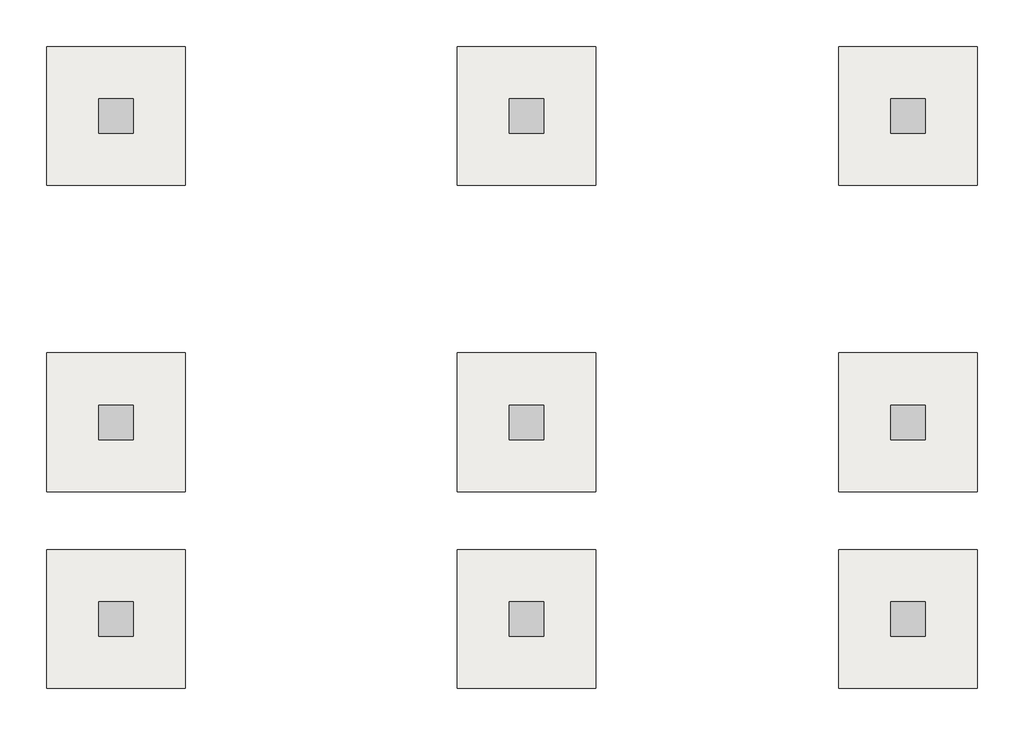
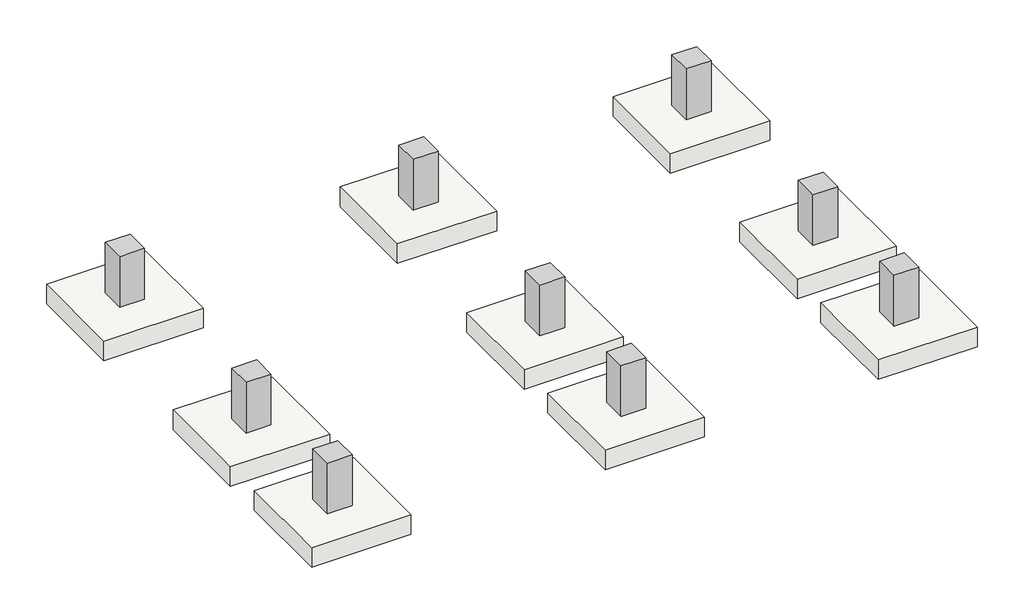
# Not in any storey: 9 columns, 9 slabs.
"""IFC4 building model written with IfcOpenShell, lengths in millimetres."""

import ifcopenshell
import ifcopenshell.guid

model = None  # the IFC model being written
_history = None  # IfcOwnerHistory: only IFC2X3 demands one
_inside = {}  # id of a spatial element -> (the spatial element, [elements in it])
_under = {}  # id of a project, library or spatial element -> (it, [spatial elements below it])
_declared = {}  # id of a project -> (the project, [libraries it declares])
_typed = {}  # id of a type object -> (the type object, [elements of that type])
_made_of = {}  # id of a material, layer set ... -> (it, [elements and type objects made of it])


def new_model(schema):
    """Start an empty IFC model of exactly this schema.

    Asked for "IFC4X3", IfcOpenShell would pick the latest addendum, in which some entities
    have other attributes; the version numbers below select the first issue.
    IFC2X3 requires an IfcOwnerHistory on every rooted entity: one is made here for all.
    """
    global model, _history
    if schema == "IFC4X3":
        model = ifcopenshell.file(schema_version=(4, 3, 0, 0))
    else:
        model = ifcopenshell.file(schema=schema)
    _inside.clear()
    _under.clear()
    _declared.clear()
    _typed.clear()
    _made_of.clear()
    _history = None
    if model.schema == "IFC2X3":
        org = make("IfcOrganization", Name="unknown")
        user = make(
            "IfcPersonAndOrganization",
            ThePerson=make("IfcPerson", FamilyName="unknown"),
            TheOrganization=org,
        )
        app = make(
            "IfcApplication",
            ApplicationDeveloper=org,
            Version="unknown",
            ApplicationFullName="unknown",
            ApplicationIdentifier="unknown",
        )
        _history = make(
            "IfcOwnerHistory",
            OwningUser=user,
            OwningApplication=app,
            ChangeAction="ADDED",
            CreationDate=0,
        )
    return model


def make(cls, **values):
    """One entity of the class cls with the attributes given. An attribute that is None is left unset."""
    return model.create_entity(
        cls, **{name: value for name, value in values.items() if value is not None}
    )


def rooted(cls, **values):
    """An entity with a GlobalId (a new one), such as an element, a storey or a relation."""
    return make(cls, GlobalId=ifcopenshell.guid.new(), OwnerHistory=_history, **values)


def si_unit(unit_type, name, prefix=None):
    """IfcSIUnit, for example si_unit("LENGTHUNIT", "METRE", prefix="MILLI")."""
    return make("IfcSIUnit", UnitType=unit_type, Prefix=prefix, Name=name)


def assignment(units):
    """IfcUnitAssignment: the units of a project."""
    return None if units is None else make("IfcUnitAssignment", Units=units)


def point(xyz):
    """IfcCartesianPoint."""
    return None if xyz is None else make("IfcCartesianPoint", Coordinates=xyz)


def direction(xyz):
    """IfcDirection."""
    return None if xyz is None else make("IfcDirection", DirectionRatios=xyz)


def frame(location, z_axis=None, x_axis=None):
    """IfcAxis2Placement3D, a coordinate frame: its origin and axes. An axis left out is left unset."""
    return make(
        "IfcAxis2Placement3D",
        Location=point(location),
        Axis=direction(z_axis),
        RefDirection=direction(x_axis),
    )


def origin():
    """The frame at (0, 0, 0) with its axes left unset."""
    return frame((0.0, 0.0, 0.0))


def place(relative_to, where):
    """IfcLocalPlacement: puts the frame where relative to a parent placement (None: the world)."""
    return make(
        "IfcLocalPlacement", PlacementRelTo=relative_to, RelativePlacement=where
    )


def context(
    kind, dimensions, precision=None, world=None, true_north=None, identifier=None
):
    """IfcGeometricRepresentationContext, for example the 3D "Model" context."""
    return make(
        "IfcGeometricRepresentationContext",
        ContextIdentifier=identifier,
        ContextType=kind,
        CoordinateSpaceDimension=dimensions,
        Precision=precision,
        WorldCoordinateSystem=world,
        TrueNorth=true_north,
    )


def project(units=None, contexts=None):
    """IfcProject with its units and contexts."""
    return rooted(
        "IfcProject",
        Name="project",
        RepresentationContexts=contexts,
        UnitsInContext=assignment(units),
    )


def spatial(cls, under=None, at=None, **own):
    """A site, building, storey or space (cls), placed at a placement, below another one or the project."""
    s = rooted(cls, ObjectPlacement=at, **own)
    if under is not None:
        _under.setdefault(under.id(), (under, []))[1].append(s)
    return s


def polyline(points):
    """IfcPolyline through the points."""
    return make("IfcPolyline", Points=[point(p) for p in points])


def outline(outer, holes=None, kind="AREA"):
    """IfcArbitraryClosedProfileDef: a profile drawn as a closed curve; with holes, ...WithVoids."""
    if holes is None:
        return make("IfcArbitraryClosedProfileDef", ProfileType=kind, OuterCurve=outer)
    return make(
        "IfcArbitraryProfileDefWithVoids",
        ProfileType=kind,
        OuterCurve=outer,
        InnerCurves=holes,
    )


def extrude(swept, where, along, depth):
    """IfcExtrudedAreaSolid: the profile swept, set in the frame where, extruded along a direction by depth."""
    return make(
        "IfcExtrudedAreaSolid",
        SweptArea=swept,
        Position=where,
        ExtrudedDirection=direction(along),
        Depth=depth,
    )


def shape(context_of_items, identifier, shape_type, items):
    """IfcShapeRepresentation: the items that make up one representation, for example the "Body"."""
    return make(
        "IfcShapeRepresentation",
        ContextOfItems=context_of_items,
        RepresentationIdentifier=identifier,
        RepresentationType=shape_type,
        Items=items,
    )


def source(mapping_origin, context_of_items, identifier, shape_type, items):
    """IfcRepresentationMap: a shape defined once, which mapped items show again and again."""
    return make(
        "IfcRepresentationMap",
        MappingOrigin=mapping_origin,
        MappedRepresentation=shape(context_of_items, identifier, shape_type, items),
    )


def transform(
    local_origin,
    x_axis=None,
    y_axis=None,
    z_axis=None,
    scale=None,
    scale2=None,
    scale3=None,
    uniform=True,
):
    """IfcCartesianTransformationOperator3D, or its non-uniform kind. x_axis, y_axis, z_axis: its Axis1, 2, 3."""
    if uniform:
        return make(
            "IfcCartesianTransformationOperator3D",
            Axis1=direction(x_axis),
            Axis2=direction(y_axis),
            LocalOrigin=point(local_origin),
            Scale=scale,
            Axis3=direction(z_axis),
        )
    return make(
        "IfcCartesianTransformationOperator3DnonUniform",
        Axis1=direction(x_axis),
        Axis2=direction(y_axis),
        LocalOrigin=point(local_origin),
        Scale=scale,
        Axis3=direction(z_axis),
        Scale2=scale2,
        Scale3=scale3,
    )


def mapped(mapping_source, mapping_target):
    """IfcMappedItem: shows the shape of a source again, moved by a transform."""
    return make(
        "IfcMappedItem", MappingSource=mapping_source, MappingTarget=mapping_target
    )


def made_of(thing, what):
    """Note that an element or type object is made of a material, layer set ...; save() writes the relation."""
    if what is not None:
        _made_of.setdefault(what.id(), (what, []))[1].append(thing)
    return thing


def element(
    cls,
    number,
    at=None,
    inside=None,
    cuts=None,
    type_object=None,
    material=None,
    context=None,
    identifier="Body",
    shape_type=None,
    held_by="IfcProductDefinitionShape",
    body=None,
    shapes=None,
    **own,
):
    """One element of the class cls, such as IfcWall. Its Tag is "e" and its number.

    at: its placement. inside: the storey or other place that contains it. cuts: it is an
    opening in that element (IfcRelVoidsElement). A single representation is given by context,
    identifier, shape_type and body (its items); several are given by shapes. held_by: the class
    of the entity that holds the representations. save() writes the other relations.
    """
    e = rooted(cls, Tag="e%d" % number, ObjectPlacement=at, **own)
    if body is not None:
        shapes = [shape(context, identifier, shape_type, body)]
    if shapes is not None:
        e.Representation = make(held_by, Representations=shapes)
    if inside is not None:
        _inside.setdefault(inside.id(), (inside, []))[1].append(e)
    if cuts is not None:
        rooted(
            "IfcRelVoidsElement", RelatingBuildingElement=cuts, RelatedOpeningElement=e
        )
    if type_object is not None:
        _typed.setdefault(type_object.id(), (type_object, []))[1].append(e)
    return made_of(e, material)


def aggregate(whole, parts):
    """IfcRelAggregates: a whole, such as a stair, and the parts it consists of."""
    return rooted("IfcRelAggregates", RelatingObject=whole, RelatedObjects=parts)


def save(model, path):
    """Write the relations noted so far, then the file.

    IfcRelAggregates (storeys below a building ...), IfcRelContainedInSpatialStructure (elements
    in a storey), IfcRelDefinesByType, IfcRelAssociatesMaterial and IfcRelDeclares: one each for
    every whole, place, type object, material and project.
    """
    for whole, parts in _under.values():
        aggregate(whole, parts)
    for where, things in _inside.values():
        rooted(
            "IfcRelContainedInSpatialStructure",
            RelatedElements=things,
            RelatingStructure=where,
        )
    for kind, things in _typed.values():
        rooted("IfcRelDefinesByType", RelatedObjects=things, RelatingType=kind)
    for what, things in _made_of.values():
        rooted("IfcRelAssociatesMaterial", RelatedObjects=things, RelatingMaterial=what)
    for by, libraries in _declared.values():
        rooted("IfcRelDeclares", RelatingContext=by, RelatedDefinitions=libraries)
    model.write(path)


def foundation_rectangular_non_pile_5fe39465(model_context):
    return source(origin(), model_context, "Body", "SweptSolid", [
        extrude(outline(polyline([(1200.0, 1200.0), (1200.0, -1200.0), (-1200.0, -1200.0), (-1200.0, 1200.0), (1200.0, 1200.0)])), frame((0.0, 0.0, -500.0), z_axis=(0.0, 0.0, 1.0), x_axis=(1.0, 0.0, 0.0)), (0.0, 0.0, 1.0), 500.0),
    ])


model = new_model("IFC4")

# Units and contexts
model_context = context("Model", 3, world=origin())
ifc_project = project(units=[si_unit("LENGTHUNIT", "METRE", prefix="MILLI")], contexts=[model_context])

# Site, building
site = spatial("IfcSite", under=ifc_project)
building = spatial("IfcBuilding", under=site)

# Columns
placement = place(None, origin())
element("IfcColumn", 1, ObjectType="RC_Column_Rectangular : H_SC_AR_S15_UG PED_W600xL600_Bit_Anchor", at=placement, inside=building, context=model_context, shape_type="SweptSolid", body=[
    extrude(outline(polyline([(300.0, 1499.5208589), (300.0, 899.5208589), (-300.0, 899.5208589), (-300.0, 1499.5208589), (300.0, 1499.5208589)])), frame((0.0, 0.0, -700.0381366), z_axis=(0.0, 0.0, 1.0), x_axis=(1.0, 0.0, 0.0)), (0.0, 0.0, 1.0), 1300.0),
])
element("IfcColumn", 2, ObjectType="RC_Column_Rectangular : H_SC_AR_S15_UG PED_W600xL600_Bit_Anchor", at=placement, inside=building, context=model_context, shape_type="SweptSolid", body=[
    extrude(outline(polyline([(7400.0, 1499.5208589), (7400.0, 899.5208589), (6800.0, 899.5208589), (6800.0, 1499.5208589), (7400.0, 1499.5208589)])), frame((0.0, 0.0, -700.0381366), z_axis=(0.0, 0.0, 1.0), x_axis=(1.0, 0.0, 0.0)), (0.0, 0.0, 1.0), 1300.0),
])
element("IfcColumn", 3, ObjectType="RC_Column_Rectangular : H_SC_AR_S15_UG PED_W600xL600_Bit_Anchor", at=placement, inside=building, context=model_context, shape_type="SweptSolid", body=[
    extrude(outline(polyline([(14000.0, 1499.5208589), (14000.0, 899.5208589), (13400.0, 899.5208589), (13400.0, 1499.5208589), (14000.0, 1499.5208589)])), frame((0.0, 0.0, -700.0381366), z_axis=(0.0, 0.0, 1.0), x_axis=(1.0, 0.0, 0.0)), (0.0, 0.0, 1.0), 1300.0),
])
element("IfcColumn", 4, ObjectType="RC_Column_Rectangular : H_SC_AR_S15_UG PED_W600xL600_Bit_Anchor", at=placement, inside=building, context=model_context, shape_type="SweptSolid", body=[
    extrude(outline(polyline([(300.0, 6799.5208589), (300.0, 6199.5208589), (-300.0, 6199.5208589), (-300.0, 6799.5208589), (300.0, 6799.5208589)])), frame((0.0, 0.0, -700.0381366), z_axis=(0.0, 0.0, 1.0), x_axis=(1.0, 0.0, 0.0)), (0.0, 0.0, 1.0), 1300.0),
])
element("IfcColumn", 5, ObjectType="RC_Column_Rectangular : H_SC_AR_S15_UG PED_W600xL600_Bit_Anchor", at=placement, inside=building, context=model_context, shape_type="SweptSolid", body=[
    extrude(outline(polyline([(7400.0, 6799.5208589), (7400.0, 6199.5208589), (6800.0, 6199.5208589), (6800.0, 6799.5208589), (7400.0, 6799.5208589)])), frame((0.0, 0.0, -700.0381366), z_axis=(0.0, 0.0, 1.0), x_axis=(1.0, 0.0, 0.0)), (0.0, 0.0, 1.0), 1300.0),
])
element("IfcColumn", 6, ObjectType="RC_Column_Rectangular : H_SC_AR_S15_UG PED_W600xL600_Bit_Anchor", at=placement, inside=building, context=model_context, shape_type="SweptSolid", body=[
    extrude(outline(polyline([(14000.0, 6799.5208589), (14000.0, 6199.5208589), (13400.0, 6199.5208589), (13400.0, 6799.5208589), (14000.0, 6799.5208589)])), frame((0.0, 0.0, -700.0381366), z_axis=(0.0, 0.0, 1.0), x_axis=(1.0, 0.0, 0.0)), (0.0, 0.0, 1.0), 1300.0),
])
element("IfcColumn", 7, ObjectType="RC_Column_Rectangular : H_SC_AR_S15_UG PED_W600xL600_Bit_Anchor", at=placement, inside=building, context=model_context, shape_type="SweptSolid", body=[
    extrude(outline(polyline([(300.0, -1900.4791411), (300.0, -2500.4791411), (-300.0, -2500.4791411), (-300.0, -1900.4791411), (300.0, -1900.4791411)])), frame((0.0, 0.0, -700.0381366), z_axis=(0.0, 0.0, 1.0), x_axis=(1.0, 0.0, 0.0)), (0.0, 0.0, 1.0), 1300.0),
])
element("IfcColumn", 8, ObjectType="RC_Column_Rectangular : H_SC_AR_S15_UG PED_W600xL600_Bit_Anchor", at=placement, inside=building, context=model_context, shape_type="SweptSolid", body=[
    extrude(outline(polyline([(7400.0, -1900.4791411), (7400.0, -2500.4791411), (6800.0, -2500.4791411), (6800.0, -1900.4791411), (7400.0, -1900.4791411)])), frame((0.0, 0.0, -700.0381366), z_axis=(0.0, 0.0, 1.0), x_axis=(1.0, 0.0, 0.0)), (0.0, 0.0, 1.0), 1300.0),
])
element("IfcColumn", 9, ObjectType="RC_Column_Rectangular : H_SC_AR_S15_UG PED_W600xL600_Bit_Anchor", at=placement, inside=building, context=model_context, shape_type="SweptSolid", body=[
    extrude(outline(polyline([(14000.0, -1900.4791411), (14000.0, -2500.4791411), (13400.0, -2500.4791411), (13400.0, -1900.4791411), (14000.0, -1900.4791411)])), frame((0.0, 0.0, -700.0381366), z_axis=(0.0, 0.0, 1.0), x_axis=(1.0, 0.0, 0.0)), (0.0, 0.0, 1.0), 1300.0),
])

# Slabs
foundation_rectangular_non_pile_shape = foundation_rectangular_non_pile_5fe39465(model_context)
element("IfcSlab", 10, ObjectType="Foundation Rectangular (Non-Pile) : H_SF_AR_S18_W2400xL2400xT500_Bitumen", at=placement, inside=building, context=model_context, shape_type="MappedRepresentation", body=[
    mapped(foundation_rectangular_non_pile_shape, transform((0.0, 1199.5208589, -700.0381366), x_axis=(1.0, 0.0, 0.0), y_axis=(0.0, 1.0, 0.0), z_axis=(0.0, 0.0, 1.0))),
])
element("IfcSlab", 11, ObjectType="Foundation Rectangular (Non-Pile) : H_SF_AR_S18_W2400xL2400xT500_Bitumen", at=placement, inside=building, context=model_context, shape_type="MappedRepresentation", body=[
    mapped(foundation_rectangular_non_pile_shape, transform((7100.0, 1199.5208589, -700.0381366), x_axis=(1.0, 0.0, 0.0), y_axis=(0.0, 1.0, 0.0), z_axis=(0.0, 0.0, 1.0))),
])
element("IfcSlab", 12, ObjectType="Foundation Rectangular (Non-Pile) : H_SF_AR_S18_W2400xL2400xT500_Bitumen", at=placement, inside=building, context=model_context, shape_type="MappedRepresentation", body=[
    mapped(foundation_rectangular_non_pile_shape, transform((13700.0, 1199.5208589, -700.0381366), x_axis=(1.0, 0.0, 0.0), y_axis=(0.0, 1.0, 0.0), z_axis=(0.0, 0.0, 1.0))),
])
element("IfcSlab", 13, ObjectType="Foundation Rectangular (Non-Pile) : H_SF_AR_S18_W2400xL2400xT500_Bitumen", at=placement, inside=building, context=model_context, shape_type="MappedRepresentation", body=[
    mapped(foundation_rectangular_non_pile_shape, transform((0.0, 6499.5208589, -700.0381366), x_axis=(1.0, 0.0, 0.0), y_axis=(0.0, 1.0, 0.0), z_axis=(0.0, 0.0, 1.0))),
])
element("IfcSlab", 14, ObjectType="Foundation Rectangular (Non-Pile) : H_SF_AR_S18_W2400xL2400xT500_Bitumen", at=placement, inside=building, context=model_context, shape_type="MappedRepresentation", body=[
    mapped(foundation_rectangular_non_pile_shape, transform((7100.0, 6499.5208589, -700.0381366), x_axis=(1.0, 0.0, 0.0), y_axis=(0.0, 1.0, 0.0), z_axis=(0.0, 0.0, 1.0))),
])
element("IfcSlab", 15, ObjectType="Foundation Rectangular (Non-Pile) : H_SF_AR_S18_W2400xL2400xT500_Bitumen", at=placement, inside=building, context=model_context, shape_type="MappedRepresentation", body=[
    mapped(foundation_rectangular_non_pile_shape, transform((13700.0, 6499.5208589, -700.0381366), x_axis=(1.0, 0.0, 0.0), y_axis=(0.0, 1.0, 0.0), z_axis=(0.0, 0.0, 1.0))),
])
element("IfcSlab", 16, ObjectType="Foundation Rectangular (Non-Pile) : H_SF_AR_S18_W2400xL2400xT500_Bitumen", at=placement, inside=building, context=model_context, shape_type="MappedRepresentation", body=[
    mapped(foundation_rectangular_non_pile_shape, transform((0.0, -2200.4791411, -700.0381366), x_axis=(1.0, 0.0, 0.0), y_axis=(0.0, 1.0, 0.0), z_axis=(0.0, 0.0, 1.0))),
])
element("IfcSlab", 17, ObjectType="Foundation Rectangular (Non-Pile) : H_SF_AR_S18_W2400xL2400xT500_Bitumen", at=placement, inside=building, context=model_context, shape_type="MappedRepresentation", body=[
    mapped(foundation_rectangular_non_pile_shape, transform((7100.0, -2200.4791411, -700.0381366), x_axis=(1.0, 0.0, 0.0), y_axis=(0.0, 1.0, 0.0), z_axis=(0.0, 0.0, 1.0))),
])
element("IfcSlab", 18, ObjectType="Foundation Rectangular (Non-Pile) : H_SF_AR_S18_W2400xL2400xT500_Bitumen", at=placement, inside=building, context=model_context, shape_type="MappedRepresentation", body=[
    mapped(foundation_rectangular_non_pile_shape, transform((13700.0, -2200.4791411, -700.0381366), x_axis=(1.0, 0.0, 0.0), y_axis=(0.0, 1.0, 0.0), z_axis=(0.0, 0.0, 1.0))),
])

save(model, "model.ifc")

# Revit data of these elements
# Type "RC_Column_Rectangular : H_SC_AR_S15_UG PED_W600xL600_Bit_Anchor"
#   Width = 600 mm
#   Length = 600 mm
#   hec_material3 [instance default] = none
#   hec_material2 [instance default] = none
#   hec_material1 [instance default] = none
#   Structural Material [instance default] = none
#   Description = (empty or 0)
# Type "Foundation Rectangular (Non-Pile) : H_SF_AR_S18_W2400xL2400xT500_Bitumen"
#   Top bar = "D25@300"
#   Description = "UG Shallow Foundation"
#   Bottom bar = "D20@300"
#   Width = 2400 mm
#   Length = 2400 mm
#   Foundation Thickness = 500 mm
#   Structural Material [instance default] = none
#   Assembly Code = ""
# Elements 1, 2, 3, 4, 5, 6, 7, 8, 9 (IfcColumn, "RC_Column_Rectangular : H_SC_AR_S15_UG PED_W600xL600_Bit_Anchor")
#   Comments = ""
#   hec_material3 = none
#   hec_material2 = none
#   hec_material1 = none
#   Structural Material = none
#   Phase Created = New Construction
# Elements 10, 11, 12, 13, 14, 15, 16, 17, 18 (IfcSlab, "Foundation Rectangular (Non-Pile) : H_SF_AR_S18_W2400xL2400xT500_Bitumen")
#   Comments = ""
#   Structural Material = none
#   Phase Created = New Construction
